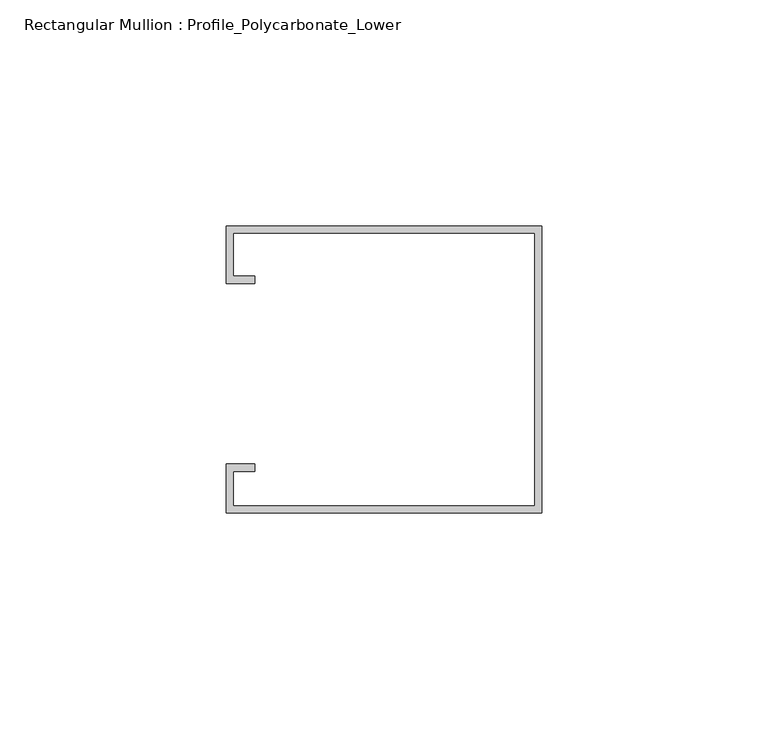
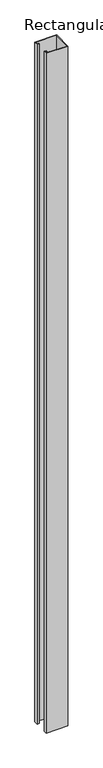
"""IFC4 building model written with IfcOpenShell, lengths in millimetres: member geometry, Rectangular Mullion : Profile_Polycarbonate_Lower."""

import ifcopenshell
import ifcopenshell.guid

model = None  # the IFC model being written
_history = None  # IfcOwnerHistory: only IFC2X3 demands one
_inside = {}  # id of a spatial element -> (the spatial element, [elements in it])
_under = {}  # id of a project, library or spatial element -> (it, [spatial elements below it])
_declared = {}  # id of a project -> (the project, [libraries it declares])
_typed = {}  # id of a type object -> (the type object, [elements of that type])
_made_of = {}  # id of a material, layer set ... -> (it, [elements and type objects made of it])


def new_model(schema):
    """Start an empty IFC model of exactly this schema.

    Asked for "IFC4X3", IfcOpenShell would pick the latest addendum, in which some entities
    have other attributes; the version numbers below select the first issue.
    IFC2X3 requires an IfcOwnerHistory on every rooted entity: one is made here for all.
    """
    global model, _history
    if schema == "IFC4X3":
        model = ifcopenshell.file(schema_version=(4, 3, 0, 0))
    else:
        model = ifcopenshell.file(schema=schema)
    _inside.clear()
    _under.clear()
    _declared.clear()
    _typed.clear()
    _made_of.clear()
    _history = None
    if model.schema == "IFC2X3":
        org = make("IfcOrganization", Name="unknown")
        user = make(
            "IfcPersonAndOrganization",
            ThePerson=make("IfcPerson", FamilyName="unknown"),
            TheOrganization=org,
        )
        app = make(
            "IfcApplication",
            ApplicationDeveloper=org,
            Version="unknown",
            ApplicationFullName="unknown",
            ApplicationIdentifier="unknown",
        )
        _history = make(
            "IfcOwnerHistory",
            OwningUser=user,
            OwningApplication=app,
            ChangeAction="ADDED",
            CreationDate=0,
        )
    return model


def make(cls, **values):
    """One entity of the class cls with the attributes given. An attribute that is None is left unset."""
    return model.create_entity(
        cls, **{name: value for name, value in values.items() if value is not None}
    )


def rooted(cls, **values):
    """An entity with a GlobalId (a new one), such as an element, a storey or a relation."""
    return make(cls, GlobalId=ifcopenshell.guid.new(), OwnerHistory=_history, **values)


def si_unit(unit_type, name, prefix=None):
    """IfcSIUnit, for example si_unit("LENGTHUNIT", "METRE", prefix="MILLI")."""
    return make("IfcSIUnit", UnitType=unit_type, Prefix=prefix, Name=name)


def assignment(units):
    """IfcUnitAssignment: the units of a project."""
    return None if units is None else make("IfcUnitAssignment", Units=units)


def point(xyz):
    """IfcCartesianPoint."""
    return None if xyz is None else make("IfcCartesianPoint", Coordinates=xyz)


def direction(xyz):
    """IfcDirection."""
    return None if xyz is None else make("IfcDirection", DirectionRatios=xyz)


def frame(location, z_axis=None, x_axis=None):
    """IfcAxis2Placement3D, a coordinate frame: its origin and axes. An axis left out is left unset."""
    return make(
        "IfcAxis2Placement3D",
        Location=point(location),
        Axis=direction(z_axis),
        RefDirection=direction(x_axis),
    )


def origin():
    """The frame at (0, 0, 0) with its axes left unset."""
    return frame((0.0, 0.0, 0.0))


def place(relative_to, where):
    """IfcLocalPlacement: puts the frame where relative to a parent placement (None: the world)."""
    return make(
        "IfcLocalPlacement", PlacementRelTo=relative_to, RelativePlacement=where
    )


def context(
    kind, dimensions, precision=None, world=None, true_north=None, identifier=None
):
    """IfcGeometricRepresentationContext, for example the 3D "Model" context."""
    return make(
        "IfcGeometricRepresentationContext",
        ContextIdentifier=identifier,
        ContextType=kind,
        CoordinateSpaceDimension=dimensions,
        Precision=precision,
        WorldCoordinateSystem=world,
        TrueNorth=true_north,
    )


def project(units=None, contexts=None):
    """IfcProject with its units and contexts."""
    return rooted(
        "IfcProject",
        Name="project",
        RepresentationContexts=contexts,
        UnitsInContext=assignment(units),
    )


def spatial(cls, under=None, at=None, **own):
    """A site, building, storey or space (cls), placed at a placement, below another one or the project."""
    s = rooted(cls, ObjectPlacement=at, **own)
    if under is not None:
        _under.setdefault(under.id(), (under, []))[1].append(s)
    return s


def polyline(points):
    """IfcPolyline through the points."""
    return make("IfcPolyline", Points=[point(p) for p in points])


def outline(outer, holes=None, kind="AREA"):
    """IfcArbitraryClosedProfileDef: a profile drawn as a closed curve; with holes, ...WithVoids."""
    if holes is None:
        return make("IfcArbitraryClosedProfileDef", ProfileType=kind, OuterCurve=outer)
    return make(
        "IfcArbitraryProfileDefWithVoids",
        ProfileType=kind,
        OuterCurve=outer,
        InnerCurves=holes,
    )


def extrude(swept, where, along, depth):
    """IfcExtrudedAreaSolid: the profile swept, set in the frame where, extruded along a direction by depth."""
    return make(
        "IfcExtrudedAreaSolid",
        SweptArea=swept,
        Position=where,
        ExtrudedDirection=direction(along),
        Depth=depth,
    )


def shape(context_of_items, identifier, shape_type, items):
    """IfcShapeRepresentation: the items that make up one representation, for example the "Body"."""
    return make(
        "IfcShapeRepresentation",
        ContextOfItems=context_of_items,
        RepresentationIdentifier=identifier,
        RepresentationType=shape_type,
        Items=items,
    )


def source(mapping_origin, context_of_items, identifier, shape_type, items):
    """IfcRepresentationMap: a shape defined once, which mapped items show again and again."""
    return make(
        "IfcRepresentationMap",
        MappingOrigin=mapping_origin,
        MappedRepresentation=shape(context_of_items, identifier, shape_type, items),
    )


def transform(
    local_origin,
    x_axis=None,
    y_axis=None,
    z_axis=None,
    scale=None,
    scale2=None,
    scale3=None,
    uniform=True,
):
    """IfcCartesianTransformationOperator3D, or its non-uniform kind. x_axis, y_axis, z_axis: its Axis1, 2, 3."""
    if uniform:
        return make(
            "IfcCartesianTransformationOperator3D",
            Axis1=direction(x_axis),
            Axis2=direction(y_axis),
            LocalOrigin=point(local_origin),
            Scale=scale,
            Axis3=direction(z_axis),
        )
    return make(
        "IfcCartesianTransformationOperator3DnonUniform",
        Axis1=direction(x_axis),
        Axis2=direction(y_axis),
        LocalOrigin=point(local_origin),
        Scale=scale,
        Axis3=direction(z_axis),
        Scale2=scale2,
        Scale3=scale3,
    )


def mapped(mapping_source, mapping_target):
    """IfcMappedItem: shows the shape of a source again, moved by a transform."""
    return make(
        "IfcMappedItem", MappingSource=mapping_source, MappingTarget=mapping_target
    )


def made_of(thing, what):
    """Note that an element or type object is made of a material, layer set ...; save() writes the relation."""
    if what is not None:
        _made_of.setdefault(what.id(), (what, []))[1].append(thing)
    return thing


def element(
    cls,
    number,
    at=None,
    inside=None,
    cuts=None,
    type_object=None,
    material=None,
    context=None,
    identifier="Body",
    shape_type=None,
    held_by="IfcProductDefinitionShape",
    body=None,
    shapes=None,
    **own,
):
    """One element of the class cls, such as IfcWall. Its Tag is "e" and its number.

    at: its placement. inside: the storey or other place that contains it. cuts: it is an
    opening in that element (IfcRelVoidsElement). A single representation is given by context,
    identifier, shape_type and body (its items); several are given by shapes. held_by: the class
    of the entity that holds the representations. save() writes the other relations.
    """
    e = rooted(cls, Tag="e%d" % number, ObjectPlacement=at, **own)
    if body is not None:
        shapes = [shape(context, identifier, shape_type, body)]
    if shapes is not None:
        e.Representation = make(held_by, Representations=shapes)
    if inside is not None:
        _inside.setdefault(inside.id(), (inside, []))[1].append(e)
    if cuts is not None:
        rooted(
            "IfcRelVoidsElement", RelatingBuildingElement=cuts, RelatedOpeningElement=e
        )
    if type_object is not None:
        _typed.setdefault(type_object.id(), (type_object, []))[1].append(e)
    return made_of(e, material)


def aggregate(whole, parts):
    """IfcRelAggregates: a whole, such as a stair, and the parts it consists of."""
    return rooted("IfcRelAggregates", RelatingObject=whole, RelatedObjects=parts)


def save(model, path):
    """Write the relations noted so far, then the file.

    IfcRelAggregates (storeys below a building ...), IfcRelContainedInSpatialStructure (elements
    in a storey), IfcRelDefinesByType, IfcRelAssociatesMaterial and IfcRelDeclares: one each for
    every whole, place, type object, material and project.
    """
    for whole, parts in _under.values():
        aggregate(whole, parts)
    for where, things in _inside.values():
        rooted(
            "IfcRelContainedInSpatialStructure",
            RelatedElements=things,
            RelatingStructure=where,
        )
    for kind, things in _typed.values():
        rooted("IfcRelDefinesByType", RelatedObjects=things, RelatingType=kind)
    for what, things in _made_of.values():
        rooted("IfcRelAssociatesMaterial", RelatedObjects=things, RelatingMaterial=what)
    for by, libraries in _declared.values():
        rooted("IfcRelDeclares", RelatingContext=by, RelatedDefinitions=libraries)
    model.write(path)


def rectangular_mullion_profile_polycarbonate_lower_3a4ba5bc(model_context):
    return source(origin(), model_context, "Body", "SweptSolid", [
        extrude(outline(polyline([(0.0, 32.7), (0.0, -30.8), (-69.85, -30.8), (-69.85, -20.0), (-63.5, -20.0), (-63.5, -21.5875), (-68.2625, -21.5875), (-68.2625, -29.2125), (-1.5875, -29.2125), (-1.5875, 31.1125), (-68.2625, 31.1125), (-68.2625, 21.5875), (-63.5, 21.5875), (-63.5, 20.0), (-69.85, 20.0), (-69.85, 32.7), (0.0, 32.7)])), frame((0.0, 0.0, -2317.75), z_axis=(0.0, 0.0, 1.0), x_axis=(1.0, 0.0, 0.0)), (0.0, 0.0, 1.0), 2317.75),
    ])


if __name__ == "__main__":
    model = new_model("IFC4")
    model_context = context("Model", 3, world=origin())
    ifc_project = project(units=[si_unit("LENGTHUNIT", "METRE", prefix="MILLI")], contexts=[model_context])
    site = spatial("IfcSite", under=ifc_project)
    building = spatial("IfcBuilding", under=site)
    placement = place(None, origin())
    rectangular_mullion_profile_polycarbonate_lower_shape = rectangular_mullion_profile_polycarbonate_lower_3a4ba5bc(model_context)
    element("IfcMember", 1, ObjectType="Rectangular Mullion : Profile_Polycarbonate_Lower", at=placement, inside=building, context=model_context, shape_type="MappedRepresentation", body=[
        mapped(rectangular_mullion_profile_polycarbonate_lower_shape, transform((0.0, 0.0, 0.0), x_axis=(1.0, 0.0, 0.0), y_axis=(0.0, 1.0, 0.0), z_axis=(0.0, 0.0, 1.0))),
    ])
    save(model, "model.ifc")

# Revit data of these elements
# Type "Rectangular Mullion : Profile_Polycarbonate_Lower"
#   built-in parameter 1007322 = 0.208333 (stored number, unit not read)
#   built-in parameter 1007321 = 0 (stored number, unit not read)
#   built-in parameter 1007320 = 0.00520833 (stored number, unit not read)
